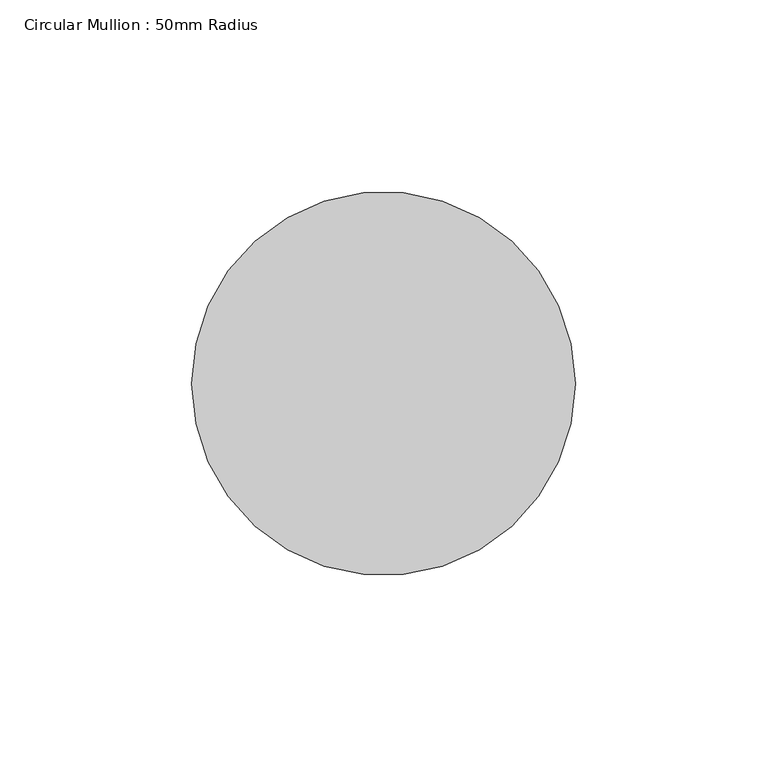
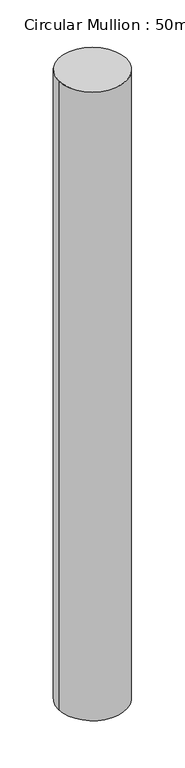
"""IFC4 building model written with IfcOpenShell, lengths in millimetres: member geometry, Circular Mullion : 50mm Radius."""

import ifcopenshell
import ifcopenshell.guid

model = None  # the IFC model being written
_history = None  # IfcOwnerHistory: only IFC2X3 demands one
_inside = {}  # id of a spatial element -> (the spatial element, [elements in it])
_under = {}  # id of a project, library or spatial element -> (it, [spatial elements below it])
_declared = {}  # id of a project -> (the project, [libraries it declares])
_typed = {}  # id of a type object -> (the type object, [elements of that type])
_made_of = {}  # id of a material, layer set ... -> (it, [elements and type objects made of it])


def new_model(schema):
    """Start an empty IFC model of exactly this schema.

    Asked for "IFC4X3", IfcOpenShell would pick the latest addendum, in which some entities
    have other attributes; the version numbers below select the first issue.
    IFC2X3 requires an IfcOwnerHistory on every rooted entity: one is made here for all.
    """
    global model, _history
    if schema == "IFC4X3":
        model = ifcopenshell.file(schema_version=(4, 3, 0, 0))
    else:
        model = ifcopenshell.file(schema=schema)
    _inside.clear()
    _under.clear()
    _declared.clear()
    _typed.clear()
    _made_of.clear()
    _history = None
    if model.schema == "IFC2X3":
        org = make("IfcOrganization", Name="unknown")
        user = make(
            "IfcPersonAndOrganization",
            ThePerson=make("IfcPerson", FamilyName="unknown"),
            TheOrganization=org,
        )
        app = make(
            "IfcApplication",
            ApplicationDeveloper=org,
            Version="unknown",
            ApplicationFullName="unknown",
            ApplicationIdentifier="unknown",
        )
        _history = make(
            "IfcOwnerHistory",
            OwningUser=user,
            OwningApplication=app,
            ChangeAction="ADDED",
            CreationDate=0,
        )
    return model


def make(cls, **values):
    """One entity of the class cls with the attributes given. An attribute that is None is left unset."""
    return model.create_entity(
        cls, **{name: value for name, value in values.items() if value is not None}
    )


def rooted(cls, **values):
    """An entity with a GlobalId (a new one), such as an element, a storey or a relation."""
    return make(cls, GlobalId=ifcopenshell.guid.new(), OwnerHistory=_history, **values)


def si_unit(unit_type, name, prefix=None):
    """IfcSIUnit, for example si_unit("LENGTHUNIT", "METRE", prefix="MILLI")."""
    return make("IfcSIUnit", UnitType=unit_type, Prefix=prefix, Name=name)


def assignment(units):
    """IfcUnitAssignment: the units of a project."""
    return None if units is None else make("IfcUnitAssignment", Units=units)


def point(xyz):
    """IfcCartesianPoint."""
    return None if xyz is None else make("IfcCartesianPoint", Coordinates=xyz)


def direction(xyz):
    """IfcDirection."""
    return None if xyz is None else make("IfcDirection", DirectionRatios=xyz)


def frame(location, z_axis=None, x_axis=None):
    """IfcAxis2Placement3D, a coordinate frame: its origin and axes. An axis left out is left unset."""
    return make(
        "IfcAxis2Placement3D",
        Location=point(location),
        Axis=direction(z_axis),
        RefDirection=direction(x_axis),
    )


def frame_2d(location, x_axis=None):
    """IfcAxis2Placement2D, a coordinate frame in the plane: its origin and x axis."""
    return make(
        "IfcAxis2Placement2D", Location=point(location), RefDirection=direction(x_axis)
    )


def origin():
    """The frame at (0, 0, 0) with its axes left unset."""
    return frame((0.0, 0.0, 0.0))


def origin_2d():
    """The frame at (0, 0) in the plane with its x axis left unset."""
    return frame_2d((0.0, 0.0))


def place(relative_to, where):
    """IfcLocalPlacement: puts the frame where relative to a parent placement (None: the world)."""
    return make(
        "IfcLocalPlacement", PlacementRelTo=relative_to, RelativePlacement=where
    )


def context(
    kind, dimensions, precision=None, world=None, true_north=None, identifier=None
):
    """IfcGeometricRepresentationContext, for example the 3D "Model" context."""
    return make(
        "IfcGeometricRepresentationContext",
        ContextIdentifier=identifier,
        ContextType=kind,
        CoordinateSpaceDimension=dimensions,
        Precision=precision,
        WorldCoordinateSystem=world,
        TrueNorth=true_north,
    )


def project(units=None, contexts=None):
    """IfcProject with its units and contexts."""
    return rooted(
        "IfcProject",
        Name="project",
        RepresentationContexts=contexts,
        UnitsInContext=assignment(units),
    )


def spatial(cls, under=None, at=None, **own):
    """A site, building, storey or space (cls), placed at a placement, below another one or the project."""
    s = rooted(cls, ObjectPlacement=at, **own)
    if under is not None:
        _under.setdefault(under.id(), (under, []))[1].append(s)
    return s


def circle_curve(where, radius):
    """IfcCircle in the frame where."""
    return make("IfcCircle", Position=where, Radius=radius)


def trimmed(basis, trim1, trim2, sense, master):
    """IfcTrimmedCurve: the piece of a basis curve between two trims."""
    return make(
        "IfcTrimmedCurve",
        BasisCurve=basis,
        Trim1=trim1,
        Trim2=trim2,
        SenseAgreement=sense,
        MasterRepresentation=master,
    )


def segment(curve, same_sense, transition):
    """IfcCompositeCurveSegment."""
    return make(
        "IfcCompositeCurveSegment",
        Transition=transition,
        SameSense=same_sense,
        ParentCurve=curve,
    )


def composite_curve(segments, self_intersect=None):
    """IfcCompositeCurve: segments joined end to end."""
    return make("IfcCompositeCurve", Segments=segments, SelfIntersect=self_intersect)


def outline(outer, holes=None, kind="AREA"):
    """IfcArbitraryClosedProfileDef: a profile drawn as a closed curve; with holes, ...WithVoids."""
    if holes is None:
        return make("IfcArbitraryClosedProfileDef", ProfileType=kind, OuterCurve=outer)
    return make(
        "IfcArbitraryProfileDefWithVoids",
        ProfileType=kind,
        OuterCurve=outer,
        InnerCurves=holes,
    )


def extrude(swept, where, along, depth):
    """IfcExtrudedAreaSolid: the profile swept, set in the frame where, extruded along a direction by depth."""
    return make(
        "IfcExtrudedAreaSolid",
        SweptArea=swept,
        Position=where,
        ExtrudedDirection=direction(along),
        Depth=depth,
    )


def shape(context_of_items, identifier, shape_type, items):
    """IfcShapeRepresentation: the items that make up one representation, for example the "Body"."""
    return make(
        "IfcShapeRepresentation",
        ContextOfItems=context_of_items,
        RepresentationIdentifier=identifier,
        RepresentationType=shape_type,
        Items=items,
    )


def source(mapping_origin, context_of_items, identifier, shape_type, items):
    """IfcRepresentationMap: a shape defined once, which mapped items show again and again."""
    return make(
        "IfcRepresentationMap",
        MappingOrigin=mapping_origin,
        MappedRepresentation=shape(context_of_items, identifier, shape_type, items),
    )


def transform(
    local_origin,
    x_axis=None,
    y_axis=None,
    z_axis=None,
    scale=None,
    scale2=None,
    scale3=None,
    uniform=True,
):
    """IfcCartesianTransformationOperator3D, or its non-uniform kind. x_axis, y_axis, z_axis: its Axis1, 2, 3."""
    if uniform:
        return make(
            "IfcCartesianTransformationOperator3D",
            Axis1=direction(x_axis),
            Axis2=direction(y_axis),
            LocalOrigin=point(local_origin),
            Scale=scale,
            Axis3=direction(z_axis),
        )
    return make(
        "IfcCartesianTransformationOperator3DnonUniform",
        Axis1=direction(x_axis),
        Axis2=direction(y_axis),
        LocalOrigin=point(local_origin),
        Scale=scale,
        Axis3=direction(z_axis),
        Scale2=scale2,
        Scale3=scale3,
    )


def mapped(mapping_source, mapping_target):
    """IfcMappedItem: shows the shape of a source again, moved by a transform."""
    return make(
        "IfcMappedItem", MappingSource=mapping_source, MappingTarget=mapping_target
    )


def made_of(thing, what):
    """Note that an element or type object is made of a material, layer set ...; save() writes the relation."""
    if what is not None:
        _made_of.setdefault(what.id(), (what, []))[1].append(thing)
    return thing


def element(
    cls,
    number,
    at=None,
    inside=None,
    cuts=None,
    type_object=None,
    material=None,
    context=None,
    identifier="Body",
    shape_type=None,
    held_by="IfcProductDefinitionShape",
    body=None,
    shapes=None,
    **own,
):
    """One element of the class cls, such as IfcWall. Its Tag is "e" and its number.

    at: its placement. inside: the storey or other place that contains it. cuts: it is an
    opening in that element (IfcRelVoidsElement). A single representation is given by context,
    identifier, shape_type and body (its items); several are given by shapes. held_by: the class
    of the entity that holds the representations. save() writes the other relations.
    """
    e = rooted(cls, Tag="e%d" % number, ObjectPlacement=at, **own)
    if body is not None:
        shapes = [shape(context, identifier, shape_type, body)]
    if shapes is not None:
        e.Representation = make(held_by, Representations=shapes)
    if inside is not None:
        _inside.setdefault(inside.id(), (inside, []))[1].append(e)
    if cuts is not None:
        rooted(
            "IfcRelVoidsElement", RelatingBuildingElement=cuts, RelatedOpeningElement=e
        )
    if type_object is not None:
        _typed.setdefault(type_object.id(), (type_object, []))[1].append(e)
    return made_of(e, material)


def aggregate(whole, parts):
    """IfcRelAggregates: a whole, such as a stair, and the parts it consists of."""
    return rooted("IfcRelAggregates", RelatingObject=whole, RelatedObjects=parts)


def save(model, path):
    """Write the relations noted so far, then the file.

    IfcRelAggregates (storeys below a building ...), IfcRelContainedInSpatialStructure (elements
    in a storey), IfcRelDefinesByType, IfcRelAssociatesMaterial and IfcRelDeclares: one each for
    every whole, place, type object, material and project.
    """
    for whole, parts in _under.values():
        aggregate(whole, parts)
    for where, things in _inside.values():
        rooted(
            "IfcRelContainedInSpatialStructure",
            RelatedElements=things,
            RelatingStructure=where,
        )
    for kind, things in _typed.values():
        rooted("IfcRelDefinesByType", RelatedObjects=things, RelatingType=kind)
    for what, things in _made_of.values():
        rooted("IfcRelAssociatesMaterial", RelatedObjects=things, RelatingMaterial=what)
    for by, libraries in _declared.values():
        rooted("IfcRelDeclares", RelatingContext=by, RelatedDefinitions=libraries)
    model.write(path)


def circular_mullion_50mm_radius_31d51a6d(model_context):
    return source(origin(), model_context, "Body", "SweptSolid", [
        extrude(outline(composite_curve([segment(trimmed(circle_curve(origin_2d(), 50.0), [point((50.0, 0.0))], [point((-50.0, 0.0))], False, "CARTESIAN"), True, "CONTINUOUS"), segment(trimmed(circle_curve(origin_2d(), 50.0), [point((-50.0, 0.0))], [point((50.0, 0.0))], False, "CARTESIAN"), True, "CONTINUOUS")], self_intersect=False)), frame((0.0, 0.0, -982.5457077), z_axis=(0.0, 0.0, 1.0), x_axis=(1.0, 0.0, 0.0)), (0.0, 0.0, 1.0), 982.5457077),
    ])


if __name__ == "__main__":
    model = new_model("IFC4")
    model_context = context("Model", 3, world=origin())
    ifc_project = project(units=[si_unit("LENGTHUNIT", "METRE", prefix="MILLI")], contexts=[model_context])
    site = spatial("IfcSite", under=ifc_project)
    building = spatial("IfcBuilding", under=site)
    placement = place(None, origin())
    circular_mullion_50mm_radius_shape = circular_mullion_50mm_radius_31d51a6d(model_context)
    element("IfcMember", 1, ObjectType="Circular Mullion : 50mm Radius", at=placement, inside=building, context=model_context, shape_type="MappedRepresentation", body=[
        mapped(circular_mullion_50mm_radius_shape, transform((0.0, 0.0, 0.0), x_axis=(1.0, 0.0, 0.0), y_axis=(0.0, 1.0, 0.0), z_axis=(0.0, 0.0, 1.0))),
    ])
    save(model, "model.ifc")

# Revit data of these elements
# Type "Circular Mullion : 50mm Radius"
#   built-in parameter 1007350 = 0.164042 (stored number, unit not read)
# Element 1 (IfcMember, "Circular Mullion : 50mm Radius")
#   Materials on its faces: "Aluminium"
# Materials
#   "Aluminium": class "Metal", colour RGB 247 247 247, transparency 0, Description = "Aluminium 6061", Cost = 0
